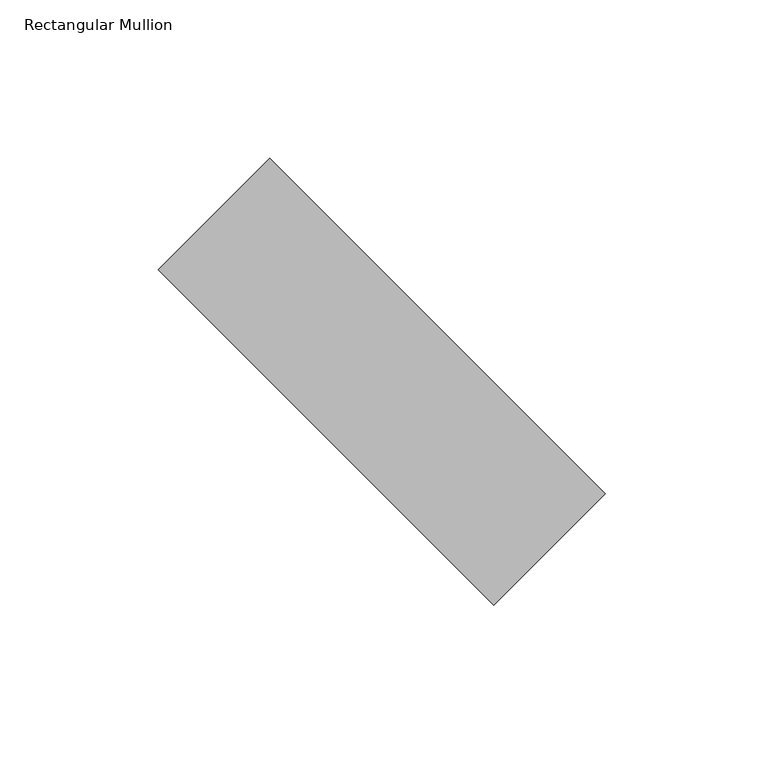
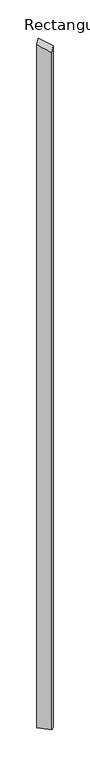
"""IFC4 building model written with IfcOpenShell, lengths in millimetres: member geometry, Rectangular Mullion : tilted mullions."""

import ifcopenshell
import ifcopenshell.guid

model = None  # the IFC model being written
_history = None  # IfcOwnerHistory: only IFC2X3 demands one
_inside = {}  # id of a spatial element -> (the spatial element, [elements in it])
_under = {}  # id of a project, library or spatial element -> (it, [spatial elements below it])
_declared = {}  # id of a project -> (the project, [libraries it declares])
_typed = {}  # id of a type object -> (the type object, [elements of that type])
_made_of = {}  # id of a material, layer set ... -> (it, [elements and type objects made of it])


def new_model(schema):
    """Start an empty IFC model of exactly this schema.

    Asked for "IFC4X3", IfcOpenShell would pick the latest addendum, in which some entities
    have other attributes; the version numbers below select the first issue.
    IFC2X3 requires an IfcOwnerHistory on every rooted entity: one is made here for all.
    """
    global model, _history
    if schema == "IFC4X3":
        model = ifcopenshell.file(schema_version=(4, 3, 0, 0))
    else:
        model = ifcopenshell.file(schema=schema)
    _inside.clear()
    _under.clear()
    _declared.clear()
    _typed.clear()
    _made_of.clear()
    _history = None
    if model.schema == "IFC2X3":
        org = make("IfcOrganization", Name="unknown")
        user = make(
            "IfcPersonAndOrganization",
            ThePerson=make("IfcPerson", FamilyName="unknown"),
            TheOrganization=org,
        )
        app = make(
            "IfcApplication",
            ApplicationDeveloper=org,
            Version="unknown",
            ApplicationFullName="unknown",
            ApplicationIdentifier="unknown",
        )
        _history = make(
            "IfcOwnerHistory",
            OwningUser=user,
            OwningApplication=app,
            ChangeAction="ADDED",
            CreationDate=0,
        )
    return model


def make(cls, **values):
    """One entity of the class cls with the attributes given. An attribute that is None is left unset."""
    return model.create_entity(
        cls, **{name: value for name, value in values.items() if value is not None}
    )


def rooted(cls, **values):
    """An entity with a GlobalId (a new one), such as an element, a storey or a relation."""
    return make(cls, GlobalId=ifcopenshell.guid.new(), OwnerHistory=_history, **values)


def si_unit(unit_type, name, prefix=None):
    """IfcSIUnit, for example si_unit("LENGTHUNIT", "METRE", prefix="MILLI")."""
    return make("IfcSIUnit", UnitType=unit_type, Prefix=prefix, Name=name)


def assignment(units):
    """IfcUnitAssignment: the units of a project."""
    return None if units is None else make("IfcUnitAssignment", Units=units)


def point(xyz):
    """IfcCartesianPoint."""
    return None if xyz is None else make("IfcCartesianPoint", Coordinates=xyz)


def direction(xyz):
    """IfcDirection."""
    return None if xyz is None else make("IfcDirection", DirectionRatios=xyz)


def frame(location, z_axis=None, x_axis=None):
    """IfcAxis2Placement3D, a coordinate frame: its origin and axes. An axis left out is left unset."""
    return make(
        "IfcAxis2Placement3D",
        Location=point(location),
        Axis=direction(z_axis),
        RefDirection=direction(x_axis),
    )


def origin():
    """The frame at (0, 0, 0) with its axes left unset."""
    return frame((0.0, 0.0, 0.0))


def place(relative_to, where):
    """IfcLocalPlacement: puts the frame where relative to a parent placement (None: the world)."""
    return make(
        "IfcLocalPlacement", PlacementRelTo=relative_to, RelativePlacement=where
    )


def context(
    kind, dimensions, precision=None, world=None, true_north=None, identifier=None
):
    """IfcGeometricRepresentationContext, for example the 3D "Model" context."""
    return make(
        "IfcGeometricRepresentationContext",
        ContextIdentifier=identifier,
        ContextType=kind,
        CoordinateSpaceDimension=dimensions,
        Precision=precision,
        WorldCoordinateSystem=world,
        TrueNorth=true_north,
    )


def project(units=None, contexts=None):
    """IfcProject with its units and contexts."""
    return rooted(
        "IfcProject",
        Name="project",
        RepresentationContexts=contexts,
        UnitsInContext=assignment(units),
    )


def spatial(cls, under=None, at=None, **own):
    """A site, building, storey or space (cls), placed at a placement, below another one or the project."""
    s = rooted(cls, ObjectPlacement=at, **own)
    if under is not None:
        _under.setdefault(under.id(), (under, []))[1].append(s)
    return s


def faces_of(points, faces, orient=None, outer=None):
    """IfcFace entities. A face is a list of loops; a loop is a list of indices into points, from 0.

    orient and outer hold one flag for each loop. By default every Orientation is true, the
    first loop of a face is its IfcFaceOuterBound and the others are IfcFaceBound.
    """
    made = []
    for i, loops in enumerate(faces):
        bounds = []
        for j, loop in enumerate(loops):
            is_outer = j == 0 if outer is None else outer[i][j]
            bounds.append(
                make(
                    "IfcFaceOuterBound" if is_outer else "IfcFaceBound",
                    Bound=make("IfcPolyLoop", Polygon=[points[k] for k in loop]),
                    Orientation=True if orient is None else orient[i][j],
                )
            )
        made.append(make("IfcFace", Bounds=bounds))
    return made


def faceted_brep(points, faces, orient=None, outer=None, voids=None):
    """IfcFacetedBrep: a solid bounded by flat faces; with voids (closed shells), ...WithVoids."""
    shared = [point(p) for p in points]
    hull = make("IfcClosedShell", CfsFaces=faces_of(shared, faces, orient, outer))
    if voids is None:
        return make("IfcFacetedBrep", Outer=hull)
    return make(
        "IfcFacetedBrepWithVoids",
        Outer=hull,
        Voids=[
            make(cls, CfsFaces=faces_of(shared, fs, o, b)) for cls, fs, o, b in voids
        ],
    )


def shape(context_of_items, identifier, shape_type, items):
    """IfcShapeRepresentation: the items that make up one representation, for example the "Body"."""
    return make(
        "IfcShapeRepresentation",
        ContextOfItems=context_of_items,
        RepresentationIdentifier=identifier,
        RepresentationType=shape_type,
        Items=items,
    )


def source(mapping_origin, context_of_items, identifier, shape_type, items):
    """IfcRepresentationMap: a shape defined once, which mapped items show again and again."""
    return make(
        "IfcRepresentationMap",
        MappingOrigin=mapping_origin,
        MappedRepresentation=shape(context_of_items, identifier, shape_type, items),
    )


def transform(
    local_origin,
    x_axis=None,
    y_axis=None,
    z_axis=None,
    scale=None,
    scale2=None,
    scale3=None,
    uniform=True,
):
    """IfcCartesianTransformationOperator3D, or its non-uniform kind. x_axis, y_axis, z_axis: its Axis1, 2, 3."""
    if uniform:
        return make(
            "IfcCartesianTransformationOperator3D",
            Axis1=direction(x_axis),
            Axis2=direction(y_axis),
            LocalOrigin=point(local_origin),
            Scale=scale,
            Axis3=direction(z_axis),
        )
    return make(
        "IfcCartesianTransformationOperator3DnonUniform",
        Axis1=direction(x_axis),
        Axis2=direction(y_axis),
        LocalOrigin=point(local_origin),
        Scale=scale,
        Axis3=direction(z_axis),
        Scale2=scale2,
        Scale3=scale3,
    )


def mapped(mapping_source, mapping_target):
    """IfcMappedItem: shows the shape of a source again, moved by a transform."""
    return make(
        "IfcMappedItem", MappingSource=mapping_source, MappingTarget=mapping_target
    )


def made_of(thing, what):
    """Note that an element or type object is made of a material, layer set ...; save() writes the relation."""
    if what is not None:
        _made_of.setdefault(what.id(), (what, []))[1].append(thing)
    return thing


def element(
    cls,
    number,
    at=None,
    inside=None,
    cuts=None,
    type_object=None,
    material=None,
    context=None,
    identifier="Body",
    shape_type=None,
    held_by="IfcProductDefinitionShape",
    body=None,
    shapes=None,
    **own,
):
    """One element of the class cls, such as IfcWall. Its Tag is "e" and its number.

    at: its placement. inside: the storey or other place that contains it. cuts: it is an
    opening in that element (IfcRelVoidsElement). A single representation is given by context,
    identifier, shape_type and body (its items); several are given by shapes. held_by: the class
    of the entity that holds the representations. save() writes the other relations.
    """
    e = rooted(cls, Tag="e%d" % number, ObjectPlacement=at, **own)
    if body is not None:
        shapes = [shape(context, identifier, shape_type, body)]
    if shapes is not None:
        e.Representation = make(held_by, Representations=shapes)
    if inside is not None:
        _inside.setdefault(inside.id(), (inside, []))[1].append(e)
    if cuts is not None:
        rooted(
            "IfcRelVoidsElement", RelatingBuildingElement=cuts, RelatedOpeningElement=e
        )
    if type_object is not None:
        _typed.setdefault(type_object.id(), (type_object, []))[1].append(e)
    return made_of(e, material)


def aggregate(whole, parts):
    """IfcRelAggregates: a whole, such as a stair, and the parts it consists of."""
    return rooted("IfcRelAggregates", RelatingObject=whole, RelatedObjects=parts)


def save(model, path):
    """Write the relations noted so far, then the file.

    IfcRelAggregates (storeys below a building ...), IfcRelContainedInSpatialStructure (elements
    in a storey), IfcRelDefinesByType, IfcRelAssociatesMaterial and IfcRelDeclares: one each for
    every whole, place, type object, material and project.
    """
    for whole, parts in _under.values():
        aggregate(whole, parts)
    for where, things in _inside.values():
        rooted(
            "IfcRelContainedInSpatialStructure",
            RelatedElements=things,
            RelatingStructure=where,
        )
    for kind, things in _typed.values():
        rooted("IfcRelDefinesByType", RelatedObjects=things, RelatingType=kind)
    for what, things in _made_of.values():
        rooted("IfcRelAssociatesMaterial", RelatedObjects=things, RelatingMaterial=what)
    for by, libraries in _declared.values():
        rooted("IfcRelDeclares", RelatingContext=by, RelatedDefinitions=libraries)
    model.write(path)


def rectangular_mullion_bea0bdf5(model_context):
    return source(origin(), model_context, "Body", "Brep", [
        faceted_brep([(-35.3553391, 70.7106781, -7999.3358332), (70.7106781, -35.3553391, -7999.3358332), (35.3553391, -70.7106781, -7999.3358332), (-70.7106781, 35.3553391, -7999.3358332), (-70.7106781, 35.3553391, 10.0090632), (-35.3553391, 70.7106781, 55.0597182), (35.3553391, -70.7106781, -55.0597182), (70.7106781, -35.3553391, -10.0090632)], [[[0, 1, 2, 3]], [[4, 5, 0, 3]], [[6, 4, 3, 2]], [[7, 6, 2, 1]], [[5, 7, 1, 0]], [[5, 4, 6, 7]]]),
    ])


if __name__ == "__main__":
    model = new_model("IFC4")
    model_context = context("Model", 3, world=origin())
    ifc_project = project(units=[si_unit("LENGTHUNIT", "METRE", prefix="MILLI")], contexts=[model_context])
    site = spatial("IfcSite", under=ifc_project)
    building = spatial("IfcBuilding", under=site)
    placement = place(None, origin())
    rectangular_mullion_shape = rectangular_mullion_bea0bdf5(model_context)
    element("IfcMember", 1, ObjectType="Rectangular Mullion : tilted mullions", at=placement, inside=building, context=model_context, shape_type="MappedRepresentation", body=[
        mapped(rectangular_mullion_shape, transform((0.0, 0.0, 0.0), x_axis=(1.0, 0.0, 0.0), y_axis=(0.0, 1.0, 0.0), z_axis=(0.0, 0.0, 1.0))),
    ])
    save(model, "model.ifc")

# Revit data of these elements
# Type "Rectangular Mullion : tilted mullions"
#   built-in parameter 1007304 = 0.492126 (stored number, unit not read)
#   built-in parameter 1007301 = 0.082021 (stored number, unit not read)
#   built-in parameter 1007300 = 0.082021 (stored number, unit not read)
# Element 1 (IfcMember, "Rectangular Mullion : tilted mullions")
#   Materials on its faces: "Aluminum"
# Materials
#   "Aluminum": class "Metal", colour RGB 244 244 244, transparency 0, Description = "Aluminum 6061", Cost = 0
